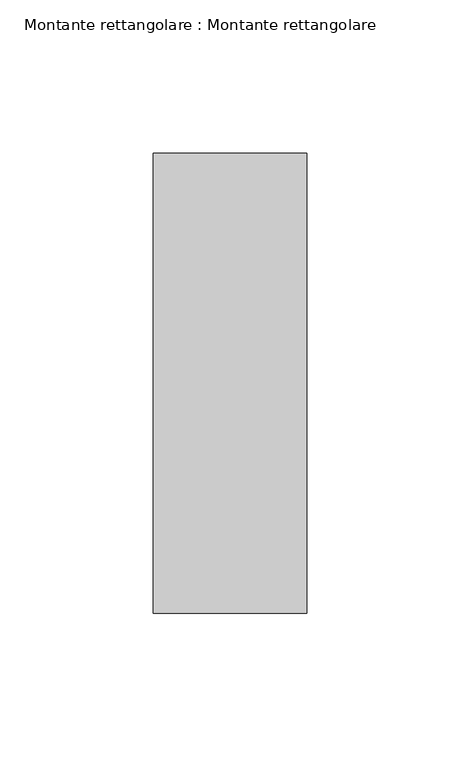
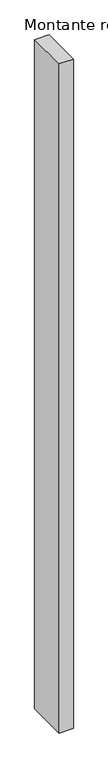
"""IFC4 building model written with IfcOpenShell, lengths in millimetres: member geometry, Montante rettangolare : Montante rettangolare."""

import ifcopenshell
import ifcopenshell.guid

model = None  # the IFC model being written
_history = None  # IfcOwnerHistory: only IFC2X3 demands one
_inside = {}  # id of a spatial element -> (the spatial element, [elements in it])
_under = {}  # id of a project, library or spatial element -> (it, [spatial elements below it])
_declared = {}  # id of a project -> (the project, [libraries it declares])
_typed = {}  # id of a type object -> (the type object, [elements of that type])
_made_of = {}  # id of a material, layer set ... -> (it, [elements and type objects made of it])


def new_model(schema):
    """Start an empty IFC model of exactly this schema.

    Asked for "IFC4X3", IfcOpenShell would pick the latest addendum, in which some entities
    have other attributes; the version numbers below select the first issue.
    IFC2X3 requires an IfcOwnerHistory on every rooted entity: one is made here for all.
    """
    global model, _history
    if schema == "IFC4X3":
        model = ifcopenshell.file(schema_version=(4, 3, 0, 0))
    else:
        model = ifcopenshell.file(schema=schema)
    _inside.clear()
    _under.clear()
    _declared.clear()
    _typed.clear()
    _made_of.clear()
    _history = None
    if model.schema == "IFC2X3":
        org = make("IfcOrganization", Name="unknown")
        user = make(
            "IfcPersonAndOrganization",
            ThePerson=make("IfcPerson", FamilyName="unknown"),
            TheOrganization=org,
        )
        app = make(
            "IfcApplication",
            ApplicationDeveloper=org,
            Version="unknown",
            ApplicationFullName="unknown",
            ApplicationIdentifier="unknown",
        )
        _history = make(
            "IfcOwnerHistory",
            OwningUser=user,
            OwningApplication=app,
            ChangeAction="ADDED",
            CreationDate=0,
        )
    return model


def make(cls, **values):
    """One entity of the class cls with the attributes given. An attribute that is None is left unset."""
    return model.create_entity(
        cls, **{name: value for name, value in values.items() if value is not None}
    )


def rooted(cls, **values):
    """An entity with a GlobalId (a new one), such as an element, a storey or a relation."""
    return make(cls, GlobalId=ifcopenshell.guid.new(), OwnerHistory=_history, **values)


def si_unit(unit_type, name, prefix=None):
    """IfcSIUnit, for example si_unit("LENGTHUNIT", "METRE", prefix="MILLI")."""
    return make("IfcSIUnit", UnitType=unit_type, Prefix=prefix, Name=name)


def assignment(units):
    """IfcUnitAssignment: the units of a project."""
    return None if units is None else make("IfcUnitAssignment", Units=units)


def point(xyz):
    """IfcCartesianPoint."""
    return None if xyz is None else make("IfcCartesianPoint", Coordinates=xyz)


def direction(xyz):
    """IfcDirection."""
    return None if xyz is None else make("IfcDirection", DirectionRatios=xyz)


def frame(location, z_axis=None, x_axis=None):
    """IfcAxis2Placement3D, a coordinate frame: its origin and axes. An axis left out is left unset."""
    return make(
        "IfcAxis2Placement3D",
        Location=point(location),
        Axis=direction(z_axis),
        RefDirection=direction(x_axis),
    )


def origin():
    """The frame at (0, 0, 0) with its axes left unset."""
    return frame((0.0, 0.0, 0.0))


def place(relative_to, where):
    """IfcLocalPlacement: puts the frame where relative to a parent placement (None: the world)."""
    return make(
        "IfcLocalPlacement", PlacementRelTo=relative_to, RelativePlacement=where
    )


def context(
    kind, dimensions, precision=None, world=None, true_north=None, identifier=None
):
    """IfcGeometricRepresentationContext, for example the 3D "Model" context."""
    return make(
        "IfcGeometricRepresentationContext",
        ContextIdentifier=identifier,
        ContextType=kind,
        CoordinateSpaceDimension=dimensions,
        Precision=precision,
        WorldCoordinateSystem=world,
        TrueNorth=true_north,
    )


def project(units=None, contexts=None):
    """IfcProject with its units and contexts."""
    return rooted(
        "IfcProject",
        Name="project",
        RepresentationContexts=contexts,
        UnitsInContext=assignment(units),
    )


def spatial(cls, under=None, at=None, **own):
    """A site, building, storey or space (cls), placed at a placement, below another one or the project."""
    s = rooted(cls, ObjectPlacement=at, **own)
    if under is not None:
        _under.setdefault(under.id(), (under, []))[1].append(s)
    return s


def polyline(points):
    """IfcPolyline through the points."""
    return make("IfcPolyline", Points=[point(p) for p in points])


def outline(outer, holes=None, kind="AREA"):
    """IfcArbitraryClosedProfileDef: a profile drawn as a closed curve; with holes, ...WithVoids."""
    if holes is None:
        return make("IfcArbitraryClosedProfileDef", ProfileType=kind, OuterCurve=outer)
    return make(
        "IfcArbitraryProfileDefWithVoids",
        ProfileType=kind,
        OuterCurve=outer,
        InnerCurves=holes,
    )


def extrude(swept, where, along, depth):
    """IfcExtrudedAreaSolid: the profile swept, set in the frame where, extruded along a direction by depth."""
    return make(
        "IfcExtrudedAreaSolid",
        SweptArea=swept,
        Position=where,
        ExtrudedDirection=direction(along),
        Depth=depth,
    )


def shape(context_of_items, identifier, shape_type, items):
    """IfcShapeRepresentation: the items that make up one representation, for example the "Body"."""
    return make(
        "IfcShapeRepresentation",
        ContextOfItems=context_of_items,
        RepresentationIdentifier=identifier,
        RepresentationType=shape_type,
        Items=items,
    )


def source(mapping_origin, context_of_items, identifier, shape_type, items):
    """IfcRepresentationMap: a shape defined once, which mapped items show again and again."""
    return make(
        "IfcRepresentationMap",
        MappingOrigin=mapping_origin,
        MappedRepresentation=shape(context_of_items, identifier, shape_type, items),
    )


def transform(
    local_origin,
    x_axis=None,
    y_axis=None,
    z_axis=None,
    scale=None,
    scale2=None,
    scale3=None,
    uniform=True,
):
    """IfcCartesianTransformationOperator3D, or its non-uniform kind. x_axis, y_axis, z_axis: its Axis1, 2, 3."""
    if uniform:
        return make(
            "IfcCartesianTransformationOperator3D",
            Axis1=direction(x_axis),
            Axis2=direction(y_axis),
            LocalOrigin=point(local_origin),
            Scale=scale,
            Axis3=direction(z_axis),
        )
    return make(
        "IfcCartesianTransformationOperator3DnonUniform",
        Axis1=direction(x_axis),
        Axis2=direction(y_axis),
        LocalOrigin=point(local_origin),
        Scale=scale,
        Axis3=direction(z_axis),
        Scale2=scale2,
        Scale3=scale3,
    )


def mapped(mapping_source, mapping_target):
    """IfcMappedItem: shows the shape of a source again, moved by a transform."""
    return make(
        "IfcMappedItem", MappingSource=mapping_source, MappingTarget=mapping_target
    )


def made_of(thing, what):
    """Note that an element or type object is made of a material, layer set ...; save() writes the relation."""
    if what is not None:
        _made_of.setdefault(what.id(), (what, []))[1].append(thing)
    return thing


def element(
    cls,
    number,
    at=None,
    inside=None,
    cuts=None,
    type_object=None,
    material=None,
    context=None,
    identifier="Body",
    shape_type=None,
    held_by="IfcProductDefinitionShape",
    body=None,
    shapes=None,
    **own,
):
    """One element of the class cls, such as IfcWall. Its Tag is "e" and its number.

    at: its placement. inside: the storey or other place that contains it. cuts: it is an
    opening in that element (IfcRelVoidsElement). A single representation is given by context,
    identifier, shape_type and body (its items); several are given by shapes. held_by: the class
    of the entity that holds the representations. save() writes the other relations.
    """
    e = rooted(cls, Tag="e%d" % number, ObjectPlacement=at, **own)
    if body is not None:
        shapes = [shape(context, identifier, shape_type, body)]
    if shapes is not None:
        e.Representation = make(held_by, Representations=shapes)
    if inside is not None:
        _inside.setdefault(inside.id(), (inside, []))[1].append(e)
    if cuts is not None:
        rooted(
            "IfcRelVoidsElement", RelatingBuildingElement=cuts, RelatedOpeningElement=e
        )
    if type_object is not None:
        _typed.setdefault(type_object.id(), (type_object, []))[1].append(e)
    return made_of(e, material)


def aggregate(whole, parts):
    """IfcRelAggregates: a whole, such as a stair, and the parts it consists of."""
    return rooted("IfcRelAggregates", RelatingObject=whole, RelatedObjects=parts)


def save(model, path):
    """Write the relations noted so far, then the file.

    IfcRelAggregates (storeys below a building ...), IfcRelContainedInSpatialStructure (elements
    in a storey), IfcRelDefinesByType, IfcRelAssociatesMaterial and IfcRelDeclares: one each for
    every whole, place, type object, material and project.
    """
    for whole, parts in _under.values():
        aggregate(whole, parts)
    for where, things in _inside.values():
        rooted(
            "IfcRelContainedInSpatialStructure",
            RelatedElements=things,
            RelatingStructure=where,
        )
    for kind, things in _typed.values():
        rooted("IfcRelDefinesByType", RelatedObjects=things, RelatingType=kind)
    for what, things in _made_of.values():
        rooted("IfcRelAssociatesMaterial", RelatedObjects=things, RelatingMaterial=what)
    for by, libraries in _declared.values():
        rooted("IfcRelDeclares", RelatingContext=by, RelatedDefinitions=libraries)
    model.write(path)


def montante_rettangolare_montante_rettangolare_4c3b9bdb(model_context):
    return source(origin(), model_context, "Body", "SweptSolid", [
        extrude(outline(polyline([(0.0, 75.0), (0.0, -75.0), (-50.0, -75.0), (-50.0, 75.0), (0.0, 75.0)])), frame((0.0, 0.0, -2500.0), z_axis=(0.0, 0.0, 1.0), x_axis=(1.0, 0.0, 0.0)), (0.0, 0.0, 1.0), 2500.0),
    ])


if __name__ == "__main__":
    model = new_model("IFC4")
    model_context = context("Model", 3, world=origin())
    ifc_project = project(units=[si_unit("LENGTHUNIT", "METRE", prefix="MILLI")], contexts=[model_context])
    site = spatial("IfcSite", under=ifc_project)
    building = spatial("IfcBuilding", under=site)
    placement = place(None, origin())
    montante_rettangolare_montante_rettangolare_shape = montante_rettangolare_montante_rettangolare_4c3b9bdb(model_context)
    element("IfcMember", 1, ObjectType="Montante rettangolare : Montante rettangolare", at=placement, inside=building, context=model_context, shape_type="MappedRepresentation", body=[
        mapped(montante_rettangolare_montante_rettangolare_shape, transform((0.0, 0.0, 0.0), x_axis=(1.0, 0.0, 0.0), y_axis=(0.0, 1.0, 0.0), z_axis=(0.0, 0.0, 1.0))),
    ])
    save(model, "model.ifc")

# Revit data of these elements
# Type "Montante rettangolare : Montante rettangolare"
#   built-in parameter 1007304 = 0.492126 (stored number, unit not read)
#   built-in parameter 1007301 = 0.082021 (stored number, unit not read)
#   built-in parameter 1007300 = 0.082021 (stored number, unit not read)
# Element 1 (IfcMember, "Montante rettangolare : Montante rettangolare")
#   Materials on its faces: "Acciaio"
# Materials
#   "Acciaio": class "Metallo", colour RGB 247 247 247, transparency 0, Description = "Acciaio, finitura zigrinata", Cost = 0
